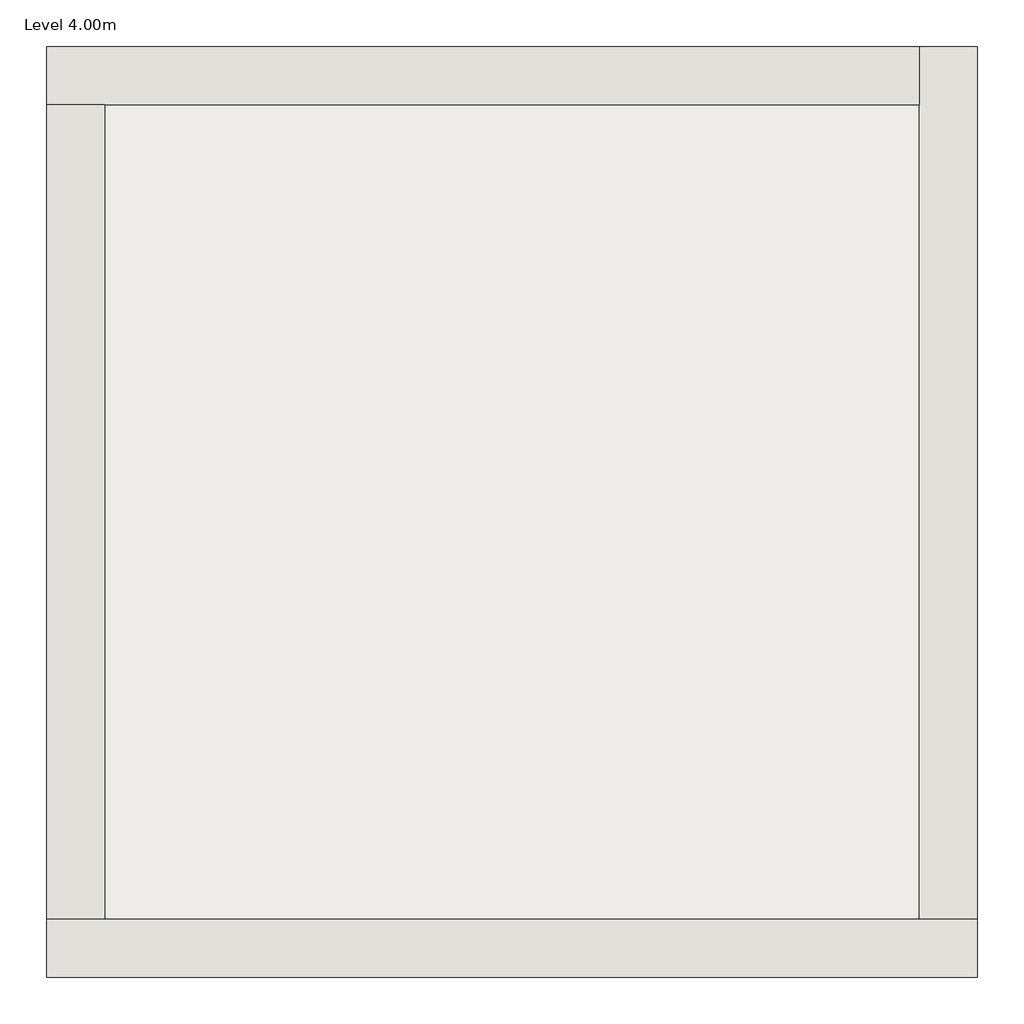
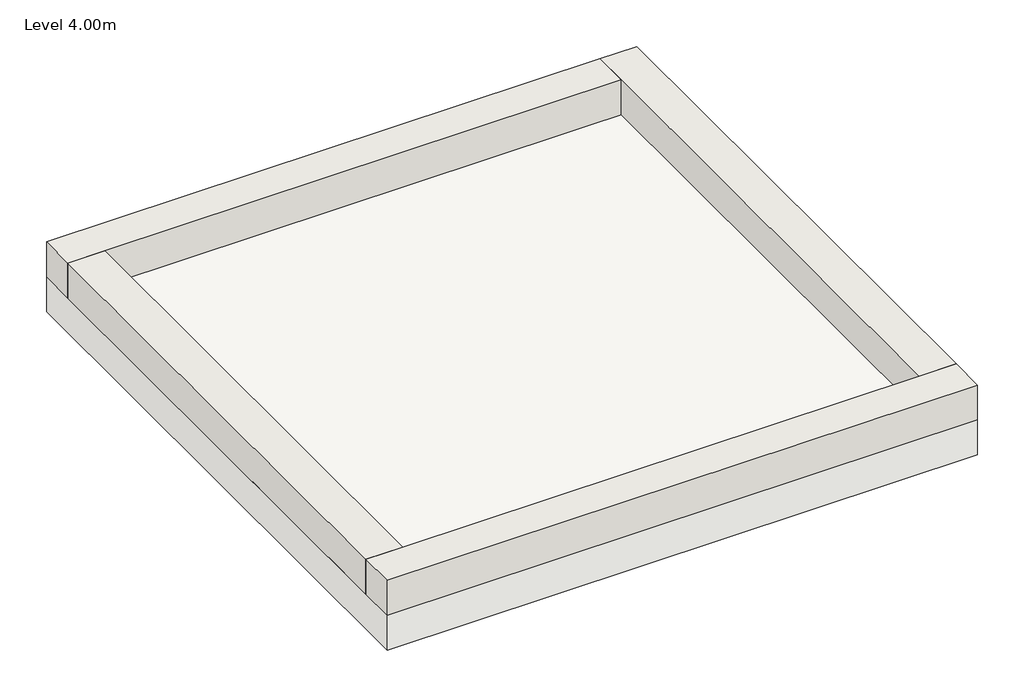
# One storey: 4 walls, 1 slab.
"""IFC4 building model written with IfcOpenShell, lengths in millimetres."""

import ifcopenshell
import ifcopenshell.guid

model = None  # the IFC model being written
_history = None  # IfcOwnerHistory: only IFC2X3 demands one
_inside = {}  # id of a spatial element -> (the spatial element, [elements in it])
_under = {}  # id of a project, library or spatial element -> (it, [spatial elements below it])
_declared = {}  # id of a project -> (the project, [libraries it declares])
_typed = {}  # id of a type object -> (the type object, [elements of that type])
_made_of = {}  # id of a material, layer set ... -> (it, [elements and type objects made of it])


def new_model(schema):
    """Start an empty IFC model of exactly this schema.

    Asked for "IFC4X3", IfcOpenShell would pick the latest addendum, in which some entities
    have other attributes; the version numbers below select the first issue.
    IFC2X3 requires an IfcOwnerHistory on every rooted entity: one is made here for all.
    """
    global model, _history
    if schema == "IFC4X3":
        model = ifcopenshell.file(schema_version=(4, 3, 0, 0))
    else:
        model = ifcopenshell.file(schema=schema)
    _inside.clear()
    _under.clear()
    _declared.clear()
    _typed.clear()
    _made_of.clear()
    _history = None
    if model.schema == "IFC2X3":
        org = make("IfcOrganization", Name="unknown")
        user = make(
            "IfcPersonAndOrganization",
            ThePerson=make("IfcPerson", FamilyName="unknown"),
            TheOrganization=org,
        )
        app = make(
            "IfcApplication",
            ApplicationDeveloper=org,
            Version="unknown",
            ApplicationFullName="unknown",
            ApplicationIdentifier="unknown",
        )
        _history = make(
            "IfcOwnerHistory",
            OwningUser=user,
            OwningApplication=app,
            ChangeAction="ADDED",
            CreationDate=0,
        )
    return model


def make(cls, **values):
    """One entity of the class cls with the attributes given. An attribute that is None is left unset."""
    return model.create_entity(
        cls, **{name: value for name, value in values.items() if value is not None}
    )


def rooted(cls, **values):
    """An entity with a GlobalId (a new one), such as an element, a storey or a relation."""
    return make(cls, GlobalId=ifcopenshell.guid.new(), OwnerHistory=_history, **values)


def si_unit(unit_type, name, prefix=None):
    """IfcSIUnit, for example si_unit("LENGTHUNIT", "METRE", prefix="MILLI")."""
    return make("IfcSIUnit", UnitType=unit_type, Prefix=prefix, Name=name)


def assignment(units):
    """IfcUnitAssignment: the units of a project."""
    return None if units is None else make("IfcUnitAssignment", Units=units)


def point(xyz):
    """IfcCartesianPoint."""
    return None if xyz is None else make("IfcCartesianPoint", Coordinates=xyz)


def direction(xyz):
    """IfcDirection."""
    return None if xyz is None else make("IfcDirection", DirectionRatios=xyz)


def frame(location, z_axis=None, x_axis=None):
    """IfcAxis2Placement3D, a coordinate frame: its origin and axes. An axis left out is left unset."""
    return make(
        "IfcAxis2Placement3D",
        Location=point(location),
        Axis=direction(z_axis),
        RefDirection=direction(x_axis),
    )


def origin():
    """The frame at (0, 0, 0) with its axes left unset."""
    return frame((0.0, 0.0, 0.0))


def place(relative_to, where):
    """IfcLocalPlacement: puts the frame where relative to a parent placement (None: the world)."""
    return make(
        "IfcLocalPlacement", PlacementRelTo=relative_to, RelativePlacement=where
    )


def context(
    kind, dimensions, precision=None, world=None, true_north=None, identifier=None
):
    """IfcGeometricRepresentationContext, for example the 3D "Model" context."""
    return make(
        "IfcGeometricRepresentationContext",
        ContextIdentifier=identifier,
        ContextType=kind,
        CoordinateSpaceDimension=dimensions,
        Precision=precision,
        WorldCoordinateSystem=world,
        TrueNorth=true_north,
    )


def project(units=None, contexts=None):
    """IfcProject with its units and contexts."""
    return rooted(
        "IfcProject",
        Name="project",
        RepresentationContexts=contexts,
        UnitsInContext=assignment(units),
    )


def spatial(cls, under=None, at=None, **own):
    """A site, building, storey or space (cls), placed at a placement, below another one or the project."""
    s = rooted(cls, ObjectPlacement=at, **own)
    if under is not None:
        _under.setdefault(under.id(), (under, []))[1].append(s)
    return s


def polyline(points):
    """IfcPolyline through the points."""
    return make("IfcPolyline", Points=[point(p) for p in points])


def outline(outer, holes=None, kind="AREA"):
    """IfcArbitraryClosedProfileDef: a profile drawn as a closed curve; with holes, ...WithVoids."""
    if holes is None:
        return make("IfcArbitraryClosedProfileDef", ProfileType=kind, OuterCurve=outer)
    return make(
        "IfcArbitraryProfileDefWithVoids",
        ProfileType=kind,
        OuterCurve=outer,
        InnerCurves=holes,
    )


def extrude(swept, where, along, depth):
    """IfcExtrudedAreaSolid: the profile swept, set in the frame where, extruded along a direction by depth."""
    return make(
        "IfcExtrudedAreaSolid",
        SweptArea=swept,
        Position=where,
        ExtrudedDirection=direction(along),
        Depth=depth,
    )


def faces_of(points, faces, orient=None, outer=None):
    """IfcFace entities. A face is a list of loops; a loop is a list of indices into points, from 0.

    orient and outer hold one flag for each loop. By default every Orientation is true, the
    first loop of a face is its IfcFaceOuterBound and the others are IfcFaceBound.
    """
    made = []
    for i, loops in enumerate(faces):
        bounds = []
        for j, loop in enumerate(loops):
            is_outer = j == 0 if outer is None else outer[i][j]
            bounds.append(
                make(
                    "IfcFaceOuterBound" if is_outer else "IfcFaceBound",
                    Bound=make("IfcPolyLoop", Polygon=[points[k] for k in loop]),
                    Orientation=True if orient is None else orient[i][j],
                )
            )
        made.append(make("IfcFace", Bounds=bounds))
    return made


def faceted_brep(points, faces, orient=None, outer=None, voids=None):
    """IfcFacetedBrep: a solid bounded by flat faces; with voids (closed shells), ...WithVoids."""
    shared = [point(p) for p in points]
    hull = make("IfcClosedShell", CfsFaces=faces_of(shared, faces, orient, outer))
    if voids is None:
        return make("IfcFacetedBrep", Outer=hull)
    return make(
        "IfcFacetedBrepWithVoids",
        Outer=hull,
        Voids=[
            make(cls, CfsFaces=faces_of(shared, fs, o, b)) for cls, fs, o, b in voids
        ],
    )


def shape(context_of_items, identifier, shape_type, items):
    """IfcShapeRepresentation: the items that make up one representation, for example the "Body"."""
    return make(
        "IfcShapeRepresentation",
        ContextOfItems=context_of_items,
        RepresentationIdentifier=identifier,
        RepresentationType=shape_type,
        Items=items,
    )


def made_of(thing, what):
    """Note that an element or type object is made of a material, layer set ...; save() writes the relation."""
    if what is not None:
        _made_of.setdefault(what.id(), (what, []))[1].append(thing)
    return thing


def element(
    cls,
    number,
    at=None,
    inside=None,
    cuts=None,
    type_object=None,
    material=None,
    context=None,
    identifier="Body",
    shape_type=None,
    held_by="IfcProductDefinitionShape",
    body=None,
    shapes=None,
    **own,
):
    """One element of the class cls, such as IfcWall. Its Tag is "e" and its number.

    at: its placement. inside: the storey or other place that contains it. cuts: it is an
    opening in that element (IfcRelVoidsElement). A single representation is given by context,
    identifier, shape_type and body (its items); several are given by shapes. held_by: the class
    of the entity that holds the representations. save() writes the other relations.
    """
    e = rooted(cls, Tag="e%d" % number, ObjectPlacement=at, **own)
    if body is not None:
        shapes = [shape(context, identifier, shape_type, body)]
    if shapes is not None:
        e.Representation = make(held_by, Representations=shapes)
    if inside is not None:
        _inside.setdefault(inside.id(), (inside, []))[1].append(e)
    if cuts is not None:
        rooted(
            "IfcRelVoidsElement", RelatingBuildingElement=cuts, RelatedOpeningElement=e
        )
    if type_object is not None:
        _typed.setdefault(type_object.id(), (type_object, []))[1].append(e)
    return made_of(e, material)


def aggregate(whole, parts):
    """IfcRelAggregates: a whole, such as a stair, and the parts it consists of."""
    return rooted("IfcRelAggregates", RelatingObject=whole, RelatedObjects=parts)


def save(model, path):
    """Write the relations noted so far, then the file.

    IfcRelAggregates (storeys below a building ...), IfcRelContainedInSpatialStructure (elements
    in a storey), IfcRelDefinesByType, IfcRelAssociatesMaterial and IfcRelDeclares: one each for
    every whole, place, type object, material and project.
    """
    for whole, parts in _under.values():
        aggregate(whole, parts)
    for where, things in _inside.values():
        rooted(
            "IfcRelContainedInSpatialStructure",
            RelatedElements=things,
            RelatingStructure=where,
        )
    for kind, things in _typed.values():
        rooted("IfcRelDefinesByType", RelatedObjects=things, RelatingType=kind)
    for what, things in _made_of.values():
        rooted("IfcRelAssociatesMaterial", RelatedObjects=things, RelatingMaterial=what)
    for by, libraries in _declared.values():
        rooted("IfcRelDeclares", RelatingContext=by, RelatedDefinitions=libraries)
    model.write(path)


model = new_model("IFC4")

# Units and contexts
model_context = context("Model", 3, world=origin())
ifc_project = project(units=[si_unit("LENGTHUNIT", "METRE", prefix="MILLI")], contexts=[model_context])

# Site, building, storey
site = spatial("IfcSite", under=ifc_project)
building = spatial("IfcBuilding", under=site)
storey = spatial("IfcBuildingStorey", under=building, Name="Level 4.00m", Elevation=4000.000128)

# Slab
placement = place(None, origin())
element("IfcSlab", 1, ObjectType="FOR INT AC-NH", at=placement, inside=storey, context=model_context, shape_type="SweptSolid", body=[
    extrude(outline(polyline([(7999.99416, 0.0), (0.0, 0.0), (0.0, 7999.99416), (7999.99416, 7999.99416), (7999.99416, 0.0)])), frame((0.0, 0.0, 3500.000112), z_axis=(0.0, 0.0, 1.0), x_axis=(1.0, 0.0, 0.0)), (0.0, 0.0, 1.0), 500.000016),
])

# Walls
element("IfcWall", 2, ObjectType="MURO EXTERIOR0.60", at=placement, inside=storey, context=model_context, shape_type="Brep", body=[
    faceted_brep([(0.0, 0.0, 4000.000128), (7999.99416, 0.0, 4000.000128), (7999.99416, 0.0, 4499.994048), (0.0, 0.0, 4499.994048), (0.0, 500.000016, 4000.000128), (0.0, 500.000016, 4499.994048), (500.000016, 500.000016, 4499.994048), (7499.994144, 500.000016, 4499.994048), (7999.99416, 500.000016, 4499.994048), (7999.99416, 500.000016, 4000.000128), (7499.994144, 500.000016, 4000.000128), (500.000016, 500.000016, 4000.000128)], [[[0, 1, 2, 3]], [[4, 5, 6, 7, 8, 9, 10, 11]], [[1, 0, 4, 11, 10, 9]], [[3, 2, 8, 7, 6, 5]], [[2, 1, 9, 8]], [[0, 3, 5, 4]]]),
])
element("IfcWall", 3, ObjectType="MURO EXTERIOR0.60", at=placement, inside=storey, context=model_context, shape_type="Brep", body=[
    faceted_brep([(7999.99416, 500.000016, 4000.000128), (7999.99416, 7999.99416, 4000.000128), (7999.99416, 7999.99416, 4499.994048), (7999.99416, 500.000016, 4499.994048), (7499.994144, 500.000016, 4000.000128), (7499.994144, 500.000016, 4499.994048), (7499.994144, 7499.994144, 4499.994048), (7499.994144, 7999.99416, 4499.994048), (7499.994144, 7999.99416, 4000.000128), (7499.994144, 7499.994144, 4000.000128)], [[[0, 1, 2, 3]], [[4, 5, 6, 7, 8, 9]], [[1, 0, 4, 9, 8]], [[3, 2, 7, 6, 5]], [[2, 1, 8, 7]], [[0, 3, 5, 4]]]),
])
element("IfcWall", 4, ObjectType="MURO EXTERIOR0.60", at=placement, inside=storey, context=model_context, shape_type="Brep", body=[
    faceted_brep([(7499.994144, 7999.99416, 4000.000128), (0.0, 7999.99416, 4000.000128), (0.0, 7999.99416, 4499.994048), (7499.994144, 7999.99416, 4499.994048), (7499.994144, 7499.994144, 4000.000128), (7499.994144, 7499.994144, 4499.994048), (500.000016, 7499.994144, 4499.994048), (0.0, 7499.994144, 4499.994048), (0.0, 7499.994144, 4000.000128), (500.000016, 7499.994144, 4000.000128)], [[[0, 1, 2, 3]], [[4, 5, 6, 7, 8, 9]], [[1, 0, 4, 9, 8]], [[3, 2, 7, 6, 5]], [[2, 1, 8, 7]], [[0, 3, 5, 4]]]),
])
element("IfcWall", 5, ObjectType="MURO EXTERIOR0.60", at=placement, inside=storey, context=model_context, shape_type="SweptSolid", body=[
    extrude(outline(polyline([(0.0, 500.000016), (0.0, 7499.994144), (500.000016, 7499.994144), (500.000016, 500.000016), (0.0, 500.000016)])), frame((0.0, 0.0, 4000.000128), z_axis=(0.0, 0.0, 1.0), x_axis=(1.0, 0.0, 0.0)), (0.0, 0.0, 1.0), 499.99392),
])

save(model, "model.ifc")

# Revit data of these elements
# Type "FOR INT AC-NH"
#   Layers, outside or top first: 10 mm no material (function 1); 55 mm no material (function 1); 120 mm no material (function 1); 250 mm no material (function 1); 50 mm no material (function 1); 15 mm no material (function 1)
# Type "MURO EXTERIOR0.60"
#   Description = "Metal Studs with Brick over sheathing on exterior and Gypsum Wall Board (GWB) on interior, Exterior Function"
#   Assembly Code = "B2010158"
#   Type Mark = "W10"
#   Layers, outside or top first: 30 mm no material (function 1); 140 mm no material (function 1); 240 mm no material (function 1); 10 mm no material (function 1); 50 mm no material (function 1); 15 mm no material (function 1); 15 mm no material (function 1)
# Element 1 (IfcSlab, "FOR INT AC-NH")
#   Height Offset From Level = 0 mm
#   Phase Created = New Construction
# Elements 2, 3, 4, 5 (IfcWall, "MURO EXTERIOR0.60")
#   Top Offset = 0 mm
#   Base Offset = 0 mm
#   Unconnected Height = 499.994 mm
#   wall height = 499.994 mm
#   Phase Created = New Construction
#   Base Constraint = Level 4.00m
#   Materials on its faces: "Default Wall"
# Materials
#   "Default Wall": class "Miscellaneous", colour RGB 192 192 192, transparency 0, Cost = 0
